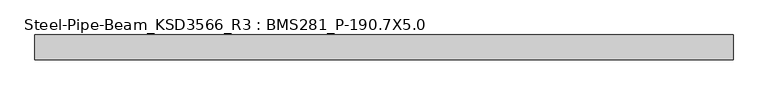
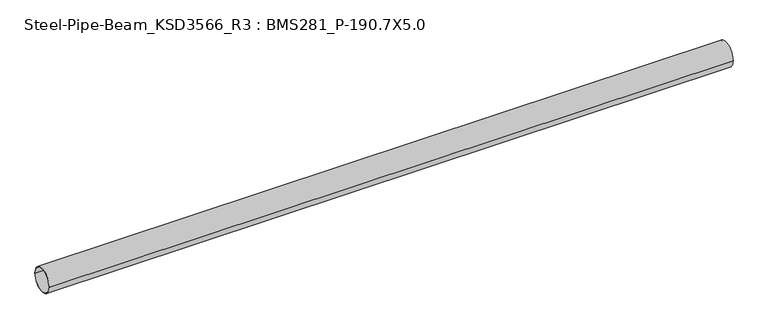
"""IFC4 building model written with IfcOpenShell, lengths in millimetres: member geometry, Steel-Pipe-Beam_KSD3566_R3 : BMS281_P-190.7X5.0."""

from ifc_helpers import new_model, si_unit, point, frame, origin, origin_2d, place, context, project, spatial, circle_curve, trimmed, segment, composite_curve, outline, extrude, source, transform, mapped, element, save


def steel_pipe_beam_ksd3566_r3_bms281_p_190_7x5_0_e6bf0e52(model_context):
    return source(origin(), model_context, "Body", "SweptSolid", [
        extrude(outline(composite_curve([segment(trimmed(circle_curve(origin_2d(), 95.35), [point((-95.35, 0.0))], [point((95.35, 0.0))], False, "CARTESIAN"), True, "CONTINUOUS"), segment(trimmed(circle_curve(origin_2d(), 95.35), [point((95.35, 0.0))], [point((-95.35, 0.0))], False, "CARTESIAN"), True, "CONTINUOUS")], self_intersect=False), holes=[composite_curve([segment(trimmed(circle_curve(origin_2d(), 90.35), [point((90.35, 0.0))], [point((-90.35, 0.0))], True, "CARTESIAN"), True, "CONTINUOUS"), segment(trimmed(circle_curve(origin_2d(), 90.35), [point((-90.35, 0.0))], [point((90.35, 0.0))], True, "CARTESIAN"), True, "CONTINUOUS")], self_intersect=False)]), frame((-2735.360064, 0.0, 0.0), z_axis=(1.0, 0.0, 0.0), x_axis=(0.0, 1.0, 0.0)), (0.0, 0.0, 1.0), 5312.4906205),
    ])


if __name__ == "__main__":
    model = new_model("IFC4")
    model_context = context("Model", 3, world=origin())
    ifc_project = project(units=[si_unit("LENGTHUNIT", "METRE", prefix="MILLI")], contexts=[model_context])
    site = spatial("IfcSite", under=ifc_project)
    building = spatial("IfcBuilding", under=site)
    placement = place(None, origin())
    steel_pipe_beam_ksd3566_r3_bms281_p_190_7x5_0_shape = steel_pipe_beam_ksd3566_r3_bms281_p_190_7x5_0_e6bf0e52(model_context)
    element("IfcMember", 1, ObjectType="Steel-Pipe-Beam_KSD3566_R3 : BMS281_P-190.7X5.0", at=placement, inside=building, context=model_context, shape_type="MappedRepresentation", body=[
        mapped(steel_pipe_beam_ksd3566_r3_bms281_p_190_7x5_0_shape, transform((0.0, 0.0, 0.0), x_axis=(1.0, 0.0, 0.0), y_axis=(0.0, 1.0, 0.0), z_axis=(0.0, 0.0, 1.0))),
    ])
    save(model, "model.ifc")

# Revit data of these elements
# Type "Steel-Pipe-Beam_KSD3566_R3 : BMS281_P-190.7X5.0"
#   Keynote = "P-190.7X5.0"
#   SteelWeight = "Light"
#   t = 0.0050 m
#   Surface Area = 0.599102 m²/m
#   Section Area = 29.1697 cm²
#   Mass per Unit Length = 22.8982 kg/m
#   Length [instance default] = 1.5000 m
#   D = 0.1907 m
#   hec_material4 [instance default] = none
#   hec_material3 [instance default] = none
#   hec_material2 [instance default] = none
#   hec_material1 [instance default] = none
#   Structural Material [instance default] = Steel, 45-345
#   Assembly Code = ""
# Element 1 (IfcMember, "Steel-Pipe-Beam_KSD3566_R3 : BMS281_P-190.7X5.0")
#   Structural Material = none
# Materials
#   "Steel, 45-345": class "Metal", colour RGB 189 187 185, transparency 0, Description = "Steel 345 MPa", Cost = 0
